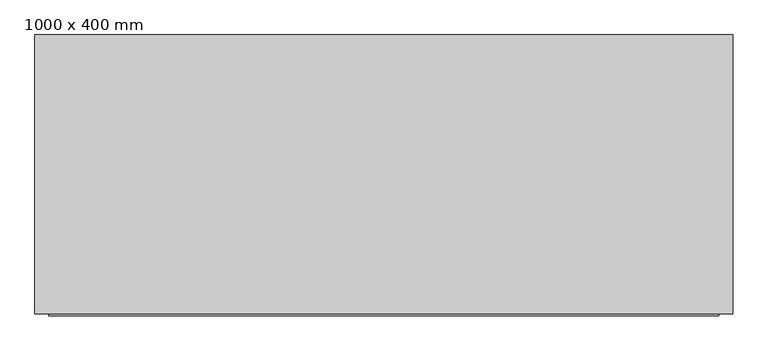
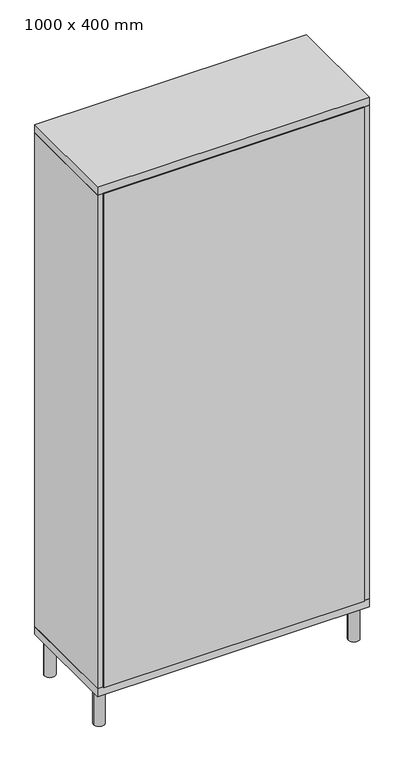
"""IFC4 building model written with IfcOpenShell, lengths in millimetres: furniture geometry, Módulo de estantería : 1000 x 400 mm."""

from ifc_helpers import new_model, si_unit, point, frame, frame_2d, origin, origin_with_axes, place, context, project, spatial, polyline, circle_curve, trimmed, segment, composite_curve, outline, extrude, source, transform, mapped, element, save


def furniture_1000_x_400_mm_ebc092ee(model_context):
    return source(origin(), model_context, "Body", "SweptSolid", [
        extrude(outline(polyline([(480.0, -191.424629), (480.0, -194.424629), (-480.0, -194.424629), (-480.0, -191.424629), (480.0, -191.424629)])), frame((0.0, 0.0, 170.0), z_axis=(0.0, 0.0, 1.0), x_axis=(1.0, 0.0, 0.0)), (0.0, 0.0, 1.0), 1920.0),
        extrude(outline(polyline([(-160.0, 180.0), (-160.0, -186.2762655), (-470.0, -186.2762655), (-470.0, 180.0), (-160.0, 180.0)])), frame((0.0, 0.0, 460.0), z_axis=(0.0, 0.0, 1.0), x_axis=(1.0, 0.0, 0.0)), (0.0, 0.0, 1.0), 10.0),
        extrude(outline(polyline([(160.0, 180.0), (160.0, -186.2762655), (-150.0, -186.2762655), (-150.0, 180.0), (160.0, 180.0)])), frame((0.0, 0.0, 460.0), z_axis=(0.0, 0.0, 1.0), x_axis=(1.0, 0.0, 0.0)), (0.0, 0.0, 1.0), 10.0),
        extrude(outline(polyline([(480.0, 180.0), (480.0, -186.2762655), (170.0, -186.2762655), (170.0, 180.0), (480.0, 180.0)])), frame((0.0, 0.0, 460.0), z_axis=(0.0, 0.0, 1.0), x_axis=(1.0, 0.0, 0.0)), (0.0, 0.0, 1.0), 10.0),
        extrude(outline(polyline([(-160.0, 180.0), (-160.0, -186.2762655), (-470.0, -186.2762655), (-470.0, 180.0), (-160.0, 180.0)])), frame((0.0, 0.0, 780.0), z_axis=(0.0, 0.0, 1.0), x_axis=(1.0, 0.0, 0.0)), (0.0, 0.0, 1.0), 10.0),
        extrude(outline(polyline([(160.0, 180.0), (160.0, -186.2762655), (-150.0, -186.2762655), (-150.0, 180.0), (160.0, 180.0)])), frame((0.0, 0.0, 780.0), z_axis=(0.0, 0.0, 1.0), x_axis=(1.0, 0.0, 0.0)), (0.0, 0.0, 1.0), 10.0),
        extrude(outline(polyline([(480.0, 180.0), (480.0, -186.2762655), (170.0, -186.2762655), (170.0, 180.0), (480.0, 180.0)])), frame((0.0, 0.0, 780.0), z_axis=(0.0, 0.0, 1.0), x_axis=(1.0, 0.0, 0.0)), (0.0, 0.0, 1.0), 10.0),
        extrude(outline(polyline([(-160.0, 180.0), (-160.0, -186.2762655), (-470.0, -186.2762655), (-470.0, 180.0), (-160.0, 180.0)])), frame((0.0, 0.0, 1450.0), z_axis=(0.0, 0.0, 1.0), x_axis=(1.0, 0.0, 0.0)), (0.0, 0.0, 1.0), 10.0),
        extrude(outline(polyline([(160.0, 180.0), (160.0, -186.2762655), (-150.0, -186.2762655), (-150.0, 180.0), (160.0, 180.0)])), frame((0.0, 0.0, 1450.0), z_axis=(0.0, 0.0, 1.0), x_axis=(1.0, 0.0, 0.0)), (0.0, 0.0, 1.0), 10.0),
        extrude(outline(polyline([(480.0, 180.0), (480.0, -186.2762655), (170.0, -186.2762655), (170.0, 180.0), (480.0, 180.0)])), frame((0.0, 0.0, 1450.0), z_axis=(0.0, 0.0, 1.0), x_axis=(1.0, 0.0, 0.0)), (0.0, 0.0, 1.0), 10.0),
        extrude(outline(polyline([(-160.0, 180.0), (-160.0, -186.2762655), (-470.0, -186.2762655), (-470.0, 180.0), (-160.0, 180.0)])), frame((0.0, 0.0, 1770.0), z_axis=(0.0, 0.0, 1.0), x_axis=(1.0, 0.0, 0.0)), (0.0, 0.0, 1.0), 10.0),
        extrude(outline(polyline([(160.0, 180.0), (160.0, -186.2762655), (-150.0, -186.2762655), (-150.0, 180.0), (160.0, 180.0)])), frame((0.0, 0.0, 1770.0), z_axis=(0.0, 0.0, 1.0), x_axis=(1.0, 0.0, 0.0)), (0.0, 0.0, 1.0), 10.0),
        extrude(outline(polyline([(480.0, 180.0), (480.0, -186.2762655), (170.0, -186.2762655), (170.0, 180.0), (480.0, 180.0)])), frame((0.0, 0.0, 1770.0), z_axis=(0.0, 0.0, 1.0), x_axis=(1.0, 0.0, 0.0)), (0.0, 0.0, 1.0), 10.0),
        extrude(outline(polyline([(170.0, 194.2277704), (170.0, -191.424629), (160.0, -191.424629), (160.0, 194.2277704), (170.0, 194.2277704)])), frame((0.0, 0.0, 170.0), z_axis=(0.0, 0.0, 1.0), x_axis=(1.0, 0.0, 0.0)), (0.0, 0.0, 1.0), 940.0),
        extrude(outline(polyline([(-150.0, 194.2277704), (-150.0, -191.424629), (-160.0, -191.424629), (-160.0, 194.2277704), (-150.0, 194.2277704)])), frame((0.0, 0.0, 170.0), z_axis=(0.0, 0.0, 1.0), x_axis=(1.0, 0.0, 0.0)), (0.0, 0.0, 1.0), 940.0),
        extrude(outline(polyline([(170.0, 194.2277704), (170.0, -191.424629), (160.0, -191.424629), (160.0, 194.2277704), (170.0, 194.2277704)])), frame((0.0, 0.0, 1140.0), z_axis=(0.0, 0.0, 1.0), x_axis=(1.0, 0.0, 0.0)), (0.0, 0.0, 1.0), 950.0),
        extrude(outline(polyline([(-150.0, 194.2277704), (-150.0, -191.424629), (-160.0, -191.424629), (-160.0, 194.2277704), (-150.0, 194.2277704)])), frame((0.0, 0.0, 1140.0), z_axis=(0.0, 0.0, 1.0), x_axis=(1.0, 0.0, 0.0)), (0.0, 0.0, 1.0), 950.0),
        extrude(outline(polyline([(480.0, 208.575371), (480.0, -191.424629), (-480.0, -191.424629), (-480.0, 208.575371), (480.0, 208.575371)])), frame((0.0, 0.0, 1110.0), z_axis=(0.0, 0.0, 1.0), x_axis=(1.0, 0.0, 0.0)), (0.0, 0.0, 1.0), 30.0),
        extrude(outline(composite_curve([segment(trimmed(circle_curve(frame_2d((-468.9411196, 166.8185459)), 20.0), [point((-448.9411196, 166.8185459))], [point((-488.9411196, 166.8185459))], False, "CARTESIAN"), True, "CONTINUOUS"), segment(trimmed(circle_curve(frame_2d((-468.9411196, 166.8185459)), 20.0), [point((-488.9411196, 166.8185459))], [point((-448.9411196, 166.8185459))], False, "CARTESIAN"), True, "CONTINUOUS")], self_intersect=False)), origin_with_axes(), (0.0, 0.0, 1.0), 140.0),
        extrude(outline(composite_curve([segment(trimmed(circle_curve(frame_2d((-468.9411196, -146.8185459)), 20.0), [point((-448.9411196, -146.8185459))], [point((-488.9411196, -146.8185459))], False, "CARTESIAN"), True, "CONTINUOUS"), segment(trimmed(circle_curve(frame_2d((-468.9411196, -146.8185459)), 20.0), [point((-488.9411196, -146.8185459))], [point((-448.9411196, -146.8185459))], False, "CARTESIAN"), True, "CONTINUOUS")], self_intersect=False)), origin_with_axes(), (0.0, 0.0, 1.0), 140.0),
        extrude(outline(composite_curve([segment(trimmed(circle_curve(frame_2d((468.9411196, 166.8185459)), 20.0), [point((448.9411196, 166.8185459))], [point((488.9411196, 166.8185459))], False, "CARTESIAN"), True, "CONTINUOUS"), segment(trimmed(circle_curve(frame_2d((468.9411196, 166.8185459)), 20.0), [point((488.9411196, 166.8185459))], [point((448.9411196, 166.8185459))], False, "CARTESIAN"), True, "CONTINUOUS")], self_intersect=False)), origin_with_axes(), (0.0, 0.0, 1.0), 140.0),
        extrude(outline(composite_curve([segment(trimmed(circle_curve(frame_2d((468.9411196, -146.8185459)), 20.0), [point((448.9411196, -146.8185459))], [point((488.9411196, -146.8185459))], False, "CARTESIAN"), True, "CONTINUOUS"), segment(trimmed(circle_curve(frame_2d((468.9411196, -146.8185459)), 20.0), [point((488.9411196, -146.8185459))], [point((448.9411196, -146.8185459))], False, "CARTESIAN"), True, "CONTINUOUS")], self_intersect=False)), origin_with_axes(), (0.0, 0.0, 1.0), 140.0),
        extrude(outline(polyline([(500.0, 208.575371), (500.0, -191.424629), (-500.0, -191.424629), (-500.0, 208.575371), (500.0, 208.575371)])), frame((0.0, 0.0, 2090.0), z_axis=(0.0, 0.0, 1.0), x_axis=(1.0, 0.0, 0.0)), (0.0, 0.0, 1.0), 30.0),
        extrude(outline(polyline([(500.0, 208.575371), (500.0, -191.424629), (-500.0, -191.424629), (-500.0, 208.575371), (500.0, 208.575371)])), frame((0.0, 0.0, 140.0), z_axis=(0.0, 0.0, 1.0), x_axis=(1.0, 0.0, 0.0)), (0.0, 0.0, 1.0), 30.0),
        extrude(outline(polyline([(-480.0, 208.575371), (-480.0, -191.424629), (-500.0, -191.424629), (-500.0, 208.575371), (-480.0, 208.575371)])), frame((0.0, 0.0, 170.0), z_axis=(0.0, 0.0, 1.0), x_axis=(1.0, 0.0, 0.0)), (0.0, 0.0, 1.0), 1920.0),
        extrude(outline(polyline([(500.0, 208.575371), (500.0, -191.424629), (480.0, -191.424629), (480.0, 208.575371), (500.0, 208.575371)])), frame((0.0, 0.0, 170.0), z_axis=(0.0, 0.0, 1.0), x_axis=(1.0, 0.0, 0.0)), (0.0, 0.0, 1.0), 1920.0),
    ])


if __name__ == "__main__":
    model = new_model("IFC4")
    model_context = context("Model", 3, world=origin())
    ifc_project = project(units=[si_unit("LENGTHUNIT", "METRE", prefix="MILLI")], contexts=[model_context])
    site = spatial("IfcSite", under=ifc_project)
    building = spatial("IfcBuilding", under=site)
    placement = place(None, origin())
    furniture_1000_x_400_mm_shape = furniture_1000_x_400_mm_ebc092ee(model_context)
    element("IfcFurniture", 1, ObjectType="Módulo de estantería : 1000 x 400 mm", at=placement, inside=building, context=model_context, shape_type="MappedRepresentation", body=[
        mapped(furniture_1000_x_400_mm_shape, transform((0.0, 0.0, 0.0), x_axis=(1.0, 0.0, 0.0), y_axis=(0.0, 1.0, 0.0), z_axis=(0.0, 0.0, 1.0))),
    ])
    save(model, "model.ifc")

# Revit data of these elements
# Type "Módulo de estantería : 1000 x 400 mm"
#   Máscara [instance default] = yes
#   Material de estructura = none
#   Material base = none
#   Material de estante = none
#   URL = ""
#   Model = ""
#   Default Elevation = 0
#   Description = (empty or 0)
#   Manufacturer = ""
#   Cost = 0
#   Assembly Code = ""
# Element 1 (IfcFurniture, "Módulo de estantería : 1000 x 400 mm")
#   Materials on its faces: "Madera - Listel"
# Materials
#   "Madera - Listel": class "Madera", colour RGB 210 180 110, transparency 0, Cost = 0
